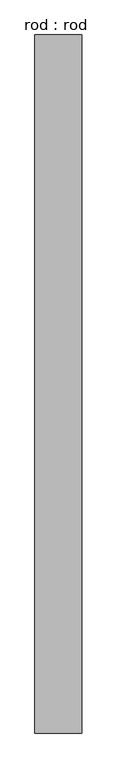
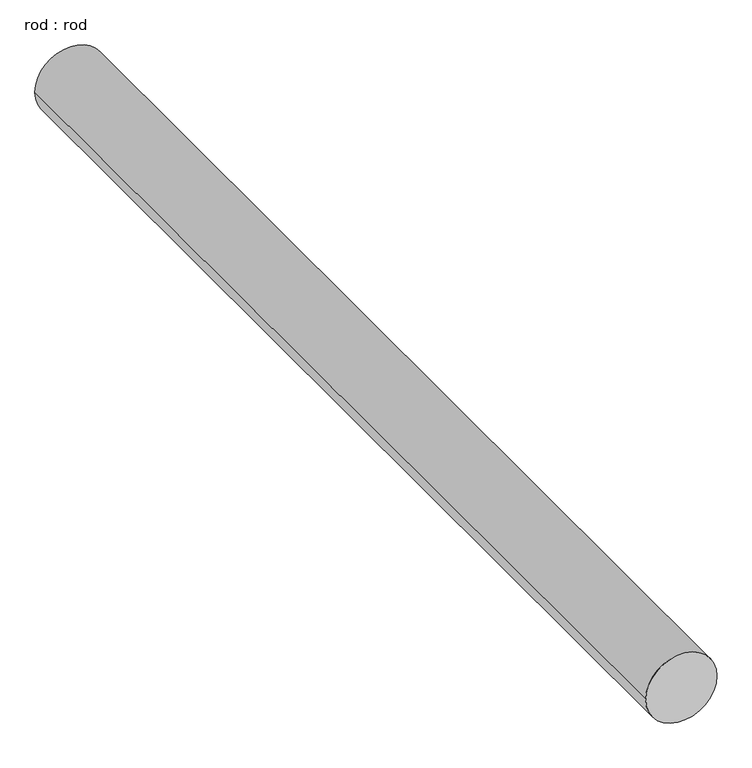
"""IFC4 building model written with IfcOpenShell, lengths in millimetres: proxy geometry, rod : rod."""

from ifc_helpers import new_model, si_unit, point, frame, frame_2d, origin, place, context, project, spatial, circle_curve, trimmed, segment, composite_curve, outline, extrude, source, transform, mapped, element, save


def rod_rod_b5d64c87(model_context):
    return source(origin(), model_context, "Body", "SweptSolid", [
        extrude(outline(composite_curve([segment(trimmed(circle_curve(frame_2d((0.0108462, 0.0)), 200.0), [point((0.0108462, 200.0))], [point((0.0108462, -200.0))], False, "CARTESIAN"), True, "CONTINUOUS"), segment(trimmed(circle_curve(frame_2d((0.0108462, 0.0)), 200.0), [point((0.0108462, -200.0))], [point((0.0108462, 200.0))], False, "CARTESIAN"), True, "CONTINUOUS")], self_intersect=False)), frame((0.0, 1119.6451643, 0.0), z_axis=(0.0, 1.0, 0.0), x_axis=(0.0, 0.0, 1.0)), (0.0, 0.0, 1.0), 5946.166902),
    ])


if __name__ == "__main__":
    model = new_model("IFC4")
    model_context = context("Model", 3, world=origin())
    ifc_project = project(units=[si_unit("LENGTHUNIT", "METRE", prefix="MILLI")], contexts=[model_context])
    site = spatial("IfcSite", under=ifc_project)
    building = spatial("IfcBuilding", under=site)
    placement = place(None, origin())
    rod_rod_shape = rod_rod_b5d64c87(model_context)
    element("IfcBuildingElementProxy", 1, Name="rod : rod", ObjectType="rod : rod", at=placement, inside=building, context=model_context, shape_type="MappedRepresentation", body=[
        mapped(rod_rod_shape, transform((0.0, 0.0, 0.0), x_axis=(1.0, 0.0, 0.0), y_axis=(0.0, 1.0, 0.0), z_axis=(0.0, 0.0, 1.0))),
    ])
    save(model, "model.ifc")

# Revit data of these elements
# Type "rod : rod"
#   Default Elevation = 0
